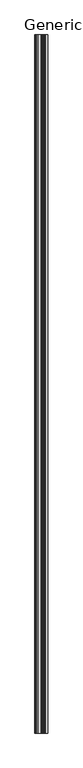
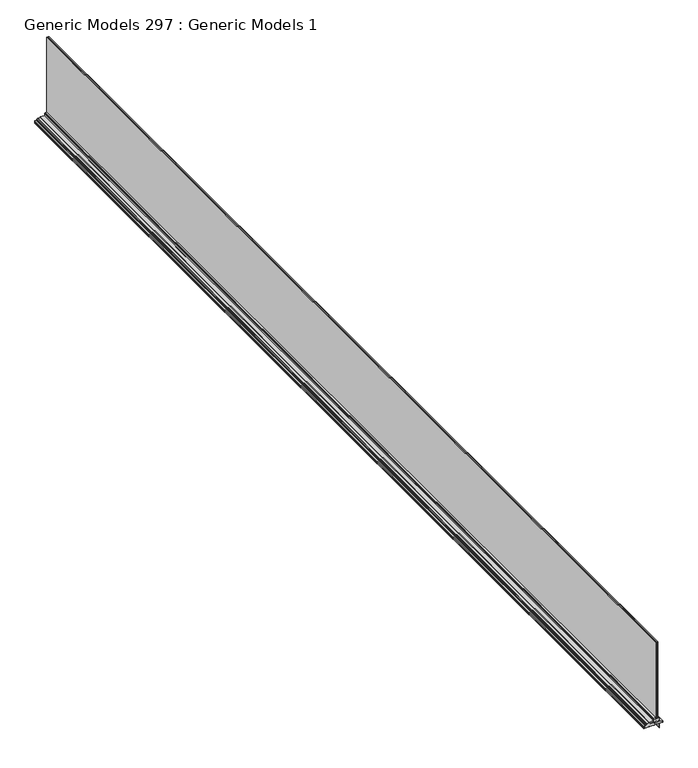
"""IFC4 building model written with IfcOpenShell, lengths in millimetres: proxy geometry, Generic Models 297 : Generic Models 1."""

from ifc_helpers import new_model, si_unit, point, frame, frame_2d, origin, place, context, project, spatial, polyline, circle_curve, trimmed, segment, composite_curve, outline, extrude, source, transform, mapped, element, save


def generic_models_297_generic_models_1_0bd4993d(model_context):
    return source(origin(), model_context, "Body", "SweptSolid", [
        extrude(outline(composite_curve([segment(polyline([(124900.2845685, 4830.4400913), (124900.2845685, 4848.5086347), (124903.4595685, 4848.5086347), (124903.4595685, 4850.7946386), (124900.2845685, 4850.7946386), (124900.2845685, 4868.3023877), (124903.4595685, 4868.3023877), (124903.4595685, 4870.5883916), (124900.2845685, 4870.5883916), (124900.2845685, 4887.6154913), (124902.3673685, 4887.6154913), (124902.3673685, 4890.7904913), (124900.2845685, 4890.7904913), (124900.2845685, 4907.8898738), (124903.4595685, 4907.8898738), (124903.4595685, 4910.1758738), (124900.2845685, 4910.1758738), (124900.2845685, 4946.6450416), (124864.9126809, 4946.6450416)]), True, "CONTINUOUS"), segment(trimmed(circle_curve(frame_2d((124864.9150218, 4947.3435419)), 0.6985041), [point((124864.9126809, 4946.6450416))], [point((124864.9174815, 4948.0420416))], False, "CARTESIAN"), True, "CONTINUOUS"), segment(polyline([(124864.9174815, 4948.0420416), (124900.2845685, 4948.0420416), (124900.2845685, 4972.929876), (124901.6815685, 4972.929876), (124901.6815685, 4966.579876), (124903.9675685, 4966.579876), (124903.9675685, 4974.4834416), (124912.8989918, 4974.4834416), (124915.3213617, 4946.6196416), (124915.3213617, 4911.6692416), (124920.1981544, 4911.6692416), (124920.1981544, 4907.6561145), (124913.7792148, 4907.6561145), (124913.7792148, 4905.6748401), (124921.7294078, 4905.6748401), (124921.7294078, 4897.2675044), (124922.6692043, 4897.2675044), (124922.6692043, 4879.7415044), (124924.9552043, 4879.7415044), (124924.9552043, 4897.2675044), (124933.6420043, 4897.2675044), (124933.6420043, 4900.3154773), (124936.8170043, 4900.3154773), (124936.8170043, 4870.9022533), (124930.4851718, 4870.9022533), (124930.4851718, 4851.8522533), (124928.0975753, 4851.8522533), (124928.0975753, 4850.2520602), (124924.9225753, 4846.3150913), (124924.9225753, 4844.7148982), (124920.9601718, 4844.7148982), (124920.9601718, 4841.5398982), (124920.1473823, 4840.7524463), (124920.1473823, 4830.4400913), (124910.2159633, 4830.4400913), (124910.2159633, 4838.3902843), (124908.2347857, 4838.3902843), (124908.2347857, 4830.4400913), (124900.2845685, 4830.4400913)]), True, "CONTINUOUS")], self_intersect=False)), frame((0.0, -1504.2676118, 0.0), z_axis=(0.0, 1.0, 0.0), x_axis=(0.0, 0.0, 1.0)), (0.0, 0.0, 1.0), 7886.7),
        extrude(outline(composite_curve([segment(polyline([(124949.1414794, 4938.1431837), (124948.1183373, 4937.1200416), (124944.5377185, 4937.1200416), (124944.5377185, 4915.6826708), (124946.9260073, 4918.0709596), (124956.8574073, 4918.0709596), (124955.8447573, 4906.2432791), (124953.6824073, 4906.2432791), (124953.6824073, 4902.4753596), (124946.1386073, 4902.4753596), (124946.1386073, 4904.0755596), (124944.5377185, 4904.0755596), (124944.5377185, 4902.1950416), (124926.2497185, 4902.1950416)]), True, "CONTINUOUS"), segment(trimmed(circle_curve(frame_2d((124926.2497185, 4903.0078416)), 0.8128), [point((124926.2497185, 4902.1950416))], [point((124925.4369185, 4903.0078416))], False, "CARTESIAN"), True, "CONTINUOUS"), segment(polyline([(124925.4369185, 4903.0078416), (124925.4369185, 4916.3428416)]), True, "CONTINUOUS"), segment(trimmed(circle_curve(frame_2d((124925.4369185, 4918.3240416)), 1.9812), [point((124925.4369185, 4916.3428416))], [point((124925.4369185, 4920.3052416))], True, "CARTESIAN"), True, "CONTINUOUS"), segment(polyline([(124925.4369185, 4920.3052416), (124925.4369185, 4932.4972416), (124920.1283185, 4932.4972416), (124920.1283185, 4938.1106416), (124928.0531185, 4938.1106416), (124928.0531185, 4940.0156416), (124924.7511185, 4940.0156416), (124924.7511185, 4941.6920416), (124922.7191185, 4941.6920416), (124922.7191185, 4944.2574416)]), True, "CONTINUOUS"), segment(trimmed(circle_curve(frame_2d((124925.1067185, 4944.2574416)), 2.3876), [point((124922.7191185, 4944.2574416))], [point((124925.1067185, 4946.6450416))], False, "CARTESIAN"), True, "CONTINUOUS"), segment(polyline([(124925.1067185, 4946.6450416), (124947.4079185, 4946.6450416), (124947.4079185, 4944.2574416), (124955.213742, 4941.7220811), (124955.4032923, 4939.2790416), (124953.3769185, 4939.2790416), (124953.3769185, 4938.1431837), (124949.1414794, 4938.1431837)]), True, "CONTINUOUS")], self_intersect=False)), frame((0.0, -1504.2676118, 0.0), z_axis=(0.0, 1.0, 0.0), x_axis=(0.0, 0.0, 1.0)), (0.0, 0.0, 1.0), 7886.7),
        extrude(outline(polyline([(4923.6272096, -1504.2676118), (4918.8647096, -1504.2676118), (4918.8647096, 6382.4323882), (4923.6272096, 6382.4323882), (4923.6272096, -1504.2676118)])), frame((0.0, 0.0, 124945.3314685), z_axis=(0.0, 0.0, 1.0), x_axis=(1.0, 0.0, 0.0)), (0.0, 0.0, 1.0), 602.3375481),
        extrude(outline(polyline([(4930.7700416, -1504.2676118), (4924.4209596, -1504.2676118), (4924.4209596, 6382.4323882), (4930.7700416, 6382.4323882), (4930.7700416, -1504.2676118)])), frame((0.0, 0.0, 124945.3314685), z_axis=(0.0, 0.0, 1.0), x_axis=(1.0, 0.0, 0.0)), (0.0, 0.0, 1.0), 6.35),
        extrude(outline(polyline([(4936.3262916, -1504.2676118), (4931.5637916, -1504.2676118), (4931.5637916, 6382.4323882), (4936.3262916, 6382.4323882), (4936.3262916, -1504.2676118)])), frame((0.0, 0.0, 124945.3314685), z_axis=(0.0, 0.0, 1.0), x_axis=(1.0, 0.0, 0.0)), (0.0, 0.0, 1.0), 602.3375481),
    ])


if __name__ == "__main__":
    model = new_model("IFC4")
    model_context = context("Model", 3, world=origin())
    ifc_project = project(units=[si_unit("LENGTHUNIT", "METRE", prefix="MILLI")], contexts=[model_context])
    site = spatial("IfcSite", under=ifc_project)
    building = spatial("IfcBuilding", under=site)
    placement = place(None, origin())
    generic_models_297_generic_models_1_shape = generic_models_297_generic_models_1_0bd4993d(model_context)
    element("IfcBuildingElementProxy", 1, Name="Generic Models 297 : Generic Models 1", ObjectType="Generic Models 297 : Generic Models 1", at=placement, inside=building, context=model_context, shape_type="MappedRepresentation", body=[
        mapped(generic_models_297_generic_models_1_shape, transform((0.0, 0.0, 0.0), x_axis=(1.0, 0.0, 0.0), y_axis=(0.0, 1.0, 0.0), z_axis=(0.0, 0.0, 1.0))),
    ])
    save(model, "model.ifc")

# Revit data of these elements
# Element 1 (IfcBuildingElementProxy, "Generic Models 297 : Generic Models 1")
#   Materials on its faces: "_WINDOW PER SCHEDULE"
# Materials
#   "_WINDOW PER SCHEDULE": class "Generic", colour RGB 255 255 255, transparency 0, Cost = 0
